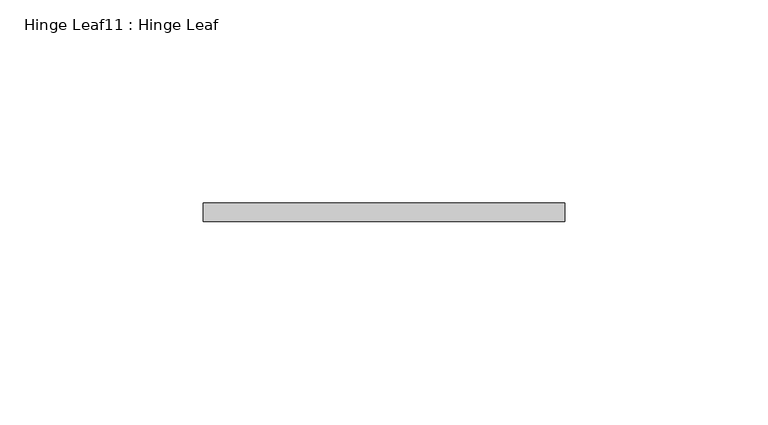
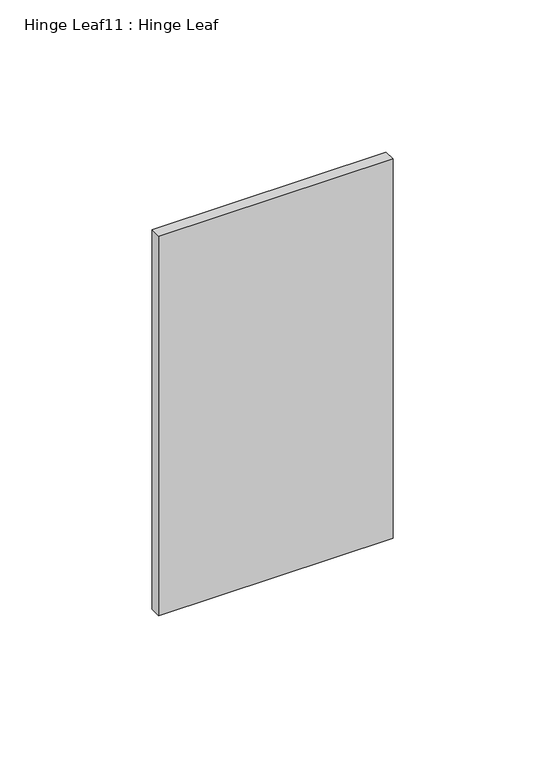
"""IFC4 building model written with IfcOpenShell, lengths in millimetres: proxy geometry, Hinge Leaf11 : Hinge Leaf."""

from ifc_helpers import new_model, si_unit, frame, origin, place, context, project, spatial, polyline, outline, extrude, source, transform, mapped, element, save


def hinge_leaf11_hinge_leaf_88ed8093(model_context):
    return source(origin(), model_context, "Body", "SweptSolid", [
        extrude(outline(polyline([(587327.7934739, -531772.5663841), (587416.6934739, -531772.5663841), (587416.6934739, -531777.1383841), (587327.7934739, -531777.1383841), (587327.7934739, -531772.5663841)])), frame((0.0, 0.0, 1123.95), z_axis=(0.0, 0.0, 1.0), x_axis=(1.0, 0.0, 0.0)), (0.0, 0.0, 1.0), 152.4),
    ])


if __name__ == "__main__":
    model = new_model("IFC4")
    model_context = context("Model", 3, world=origin())
    ifc_project = project(units=[si_unit("LENGTHUNIT", "METRE", prefix="MILLI")], contexts=[model_context])
    site = spatial("IfcSite", under=ifc_project)
    building = spatial("IfcBuilding", under=site)
    placement = place(None, origin())
    hinge_leaf11_hinge_leaf_shape = hinge_leaf11_hinge_leaf_88ed8093(model_context)
    element("IfcBuildingElementProxy", 1, Name="Hinge Leaf11 : Hinge Leaf", ObjectType="Hinge Leaf11 : Hinge Leaf", at=placement, inside=building, context=model_context, shape_type="MappedRepresentation", body=[
        mapped(hinge_leaf11_hinge_leaf_shape, transform((0.0, 0.0, 0.0), x_axis=(1.0, 0.0, 0.0), y_axis=(0.0, 1.0, 0.0), z_axis=(0.0, 0.0, 1.0))),
    ])
    save(model, "model.ifc")

# Revit data of these elements
# Element 1 (IfcBuildingElementProxy, "Hinge Leaf11 : Hinge Leaf")
#   Materials on its faces: "6\"X6\" WELD-ON STL BUTT HINGE"
# Materials
#   "6\"X6\" WELD-ON STL BUTT HINGE": class "Metal", colour RGB 189 187 185, transparency 0, Description = "Carbon steel", Cost = 0
